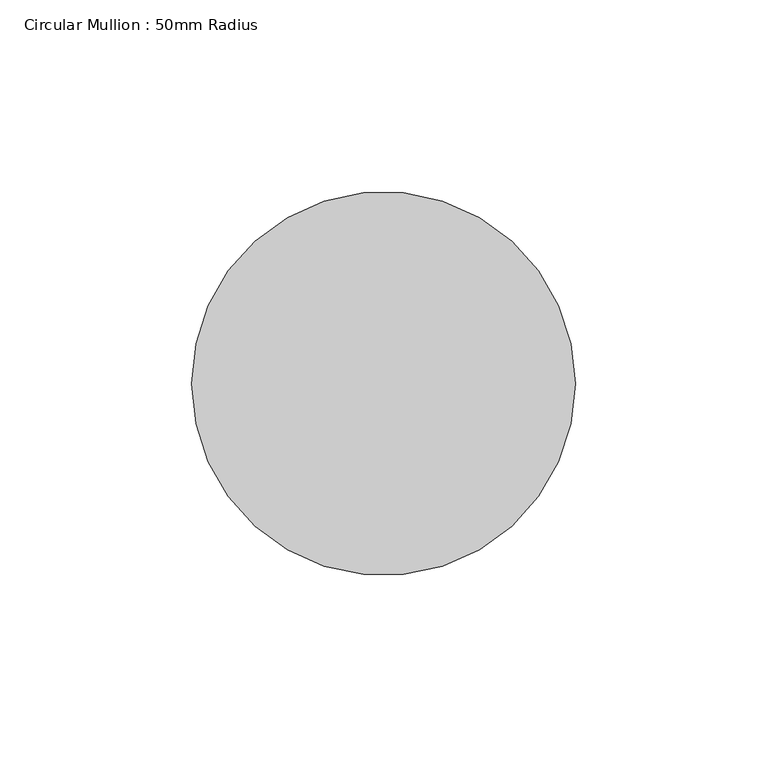
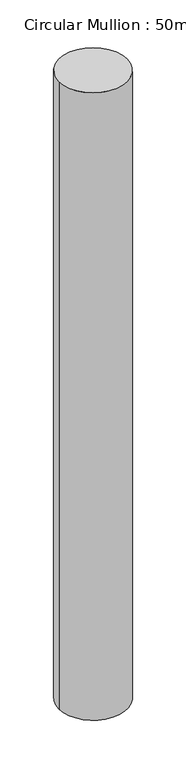
"""IFC4 building model written with IfcOpenShell, lengths in millimetres: member geometry, Circular Mullion : 50mm Radius."""

from ifc_helpers import new_model, si_unit, point, frame, origin, origin_2d, place, context, project, spatial, circle_curve, trimmed, segment, composite_curve, outline, extrude, source, transform, mapped, element, save


def circular_mullion_50mm_radius_27b52568(model_context):
    return source(origin(), model_context, "Body", "SweptSolid", [
        extrude(outline(composite_curve([segment(trimmed(circle_curve(origin_2d(), 50.0), [point((50.0, 0.0))], [point((-50.0, 0.0))], False, "CARTESIAN"), True, "CONTINUOUS"), segment(trimmed(circle_curve(origin_2d(), 50.0), [point((-50.0, 0.0))], [point((50.0, 0.0))], False, "CARTESIAN"), True, "CONTINUOUS")], self_intersect=False)), frame((0.0, 0.0, -971.8410431), z_axis=(0.0, 0.0, 1.0), x_axis=(1.0, 0.0, 0.0)), (0.0, 0.0, 1.0), 971.8410431),
    ])


if __name__ == "__main__":
    model = new_model("IFC4")
    model_context = context("Model", 3, world=origin())
    ifc_project = project(units=[si_unit("LENGTHUNIT", "METRE", prefix="MILLI")], contexts=[model_context])
    site = spatial("IfcSite", under=ifc_project)
    building = spatial("IfcBuilding", under=site)
    placement = place(None, origin())
    circular_mullion_50mm_radius_shape = circular_mullion_50mm_radius_27b52568(model_context)
    element("IfcMember", 1, ObjectType="Circular Mullion : 50mm Radius", at=placement, inside=building, context=model_context, shape_type="MappedRepresentation", body=[
        mapped(circular_mullion_50mm_radius_shape, transform((0.0, 0.0, 0.0), x_axis=(1.0, 0.0, 0.0), y_axis=(0.0, 1.0, 0.0), z_axis=(0.0, 0.0, 1.0))),
    ])
    save(model, "model.ifc")

# Revit data of these elements
# Type "Circular Mullion : 50mm Radius"
#   built-in parameter 1007350 = 0.164042 (stored number, unit not read)
# Element 1 (IfcMember, "Circular Mullion : 50mm Radius")
#   Materials on its faces: "Aluminium"
# Materials
#   "Aluminium": class "Metal", colour RGB 247 247 247, transparency 0, Description = "Aluminium 6061", Cost = 0
